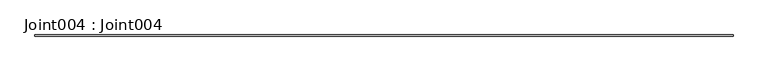
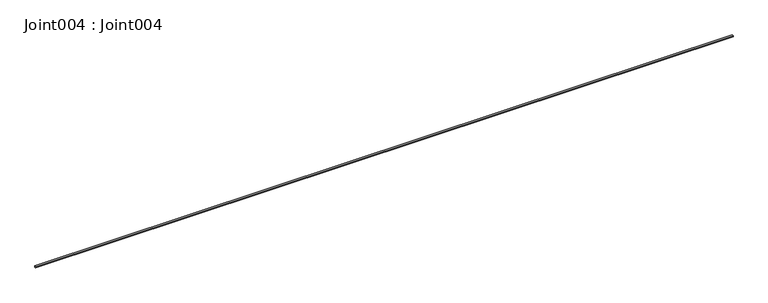
"""IFC4 building model written with IfcOpenShell, lengths in millimetres: proxy geometry, Joint004 : Joint004."""

from ifc_helpers import new_model, si_unit, point, frame, frame_2d, origin, place, context, project, spatial, polyline, circle_curve, trimmed, segment, composite_curve, outline, extrude, source, transform, mapped, element, save


def joint004_joint004_8d49f665(model_context):
    return source(origin(), model_context, "Body", "SweptSolid", [
        extrude(outline(composite_curve([segment(polyline([(10405.3793386, 40791.8007813), (10405.3793386, 40795.71875)]), True, "CONTINUOUS"), segment(trimmed(circle_curve(frame_2d((10406.9776706, 40800.890625)), 5.4132205), [point((10405.3793386, 40795.71875))], [point((10408.5760026, 40795.71875))], True, "CARTESIAN"), True, "CONTINUOUS"), segment(polyline([(10408.5760026, 40795.71875), (10408.5760026, 40791.8007813)]), True, "CONTINUOUS"), segment(trimmed(circle_curve(frame_2d((10406.9776706, 40796.9726563)), 5.4132205), [point((10408.5760026, 40791.8007813))], [point((10405.3793386, 40791.8007813))], False, "CARTESIAN"), True, "CONTINUOUS")], self_intersect=False)), frame((3694.2883192, 0.0, 0.0), z_axis=(1.0, 0.0, 0.0), x_axis=(0.0, 1.0, 0.0)), (0.0, 0.0, 1.0), 2000.0),
    ])


if __name__ == "__main__":
    model = new_model("IFC4")
    model_context = context("Model", 3, world=origin())
    ifc_project = project(units=[si_unit("LENGTHUNIT", "METRE", prefix="MILLI")], contexts=[model_context])
    site = spatial("IfcSite", under=ifc_project)
    building = spatial("IfcBuilding", under=site)
    placement = place(None, origin())
    joint004_joint004_shape = joint004_joint004_8d49f665(model_context)
    element("IfcBuildingElementProxy", 1, Name="Joint004 : Joint004", ObjectType="Joint004 : Joint004", at=placement, inside=building, context=model_context, shape_type="MappedRepresentation", body=[
        mapped(joint004_joint004_shape, transform((0.0, 0.0, 0.0), x_axis=(1.0, 0.0, 0.0), y_axis=(0.0, 1.0, 0.0), z_axis=(0.0, 0.0, 1.0))),
    ])
    save(model, "model.ifc")

# Revit data of these elements
# Type "Joint004 : Joint004"
#   NameOverride = "Joint004"
# Element 1 (IfcBuildingElementProxy, "Joint004 : Joint004")
#   Materials on its faces: "SEALANT JOINT"
# Materials
#   "SEALANT JOINT": class "Unassigned", colour RGB 142 225 148, transparency 0
